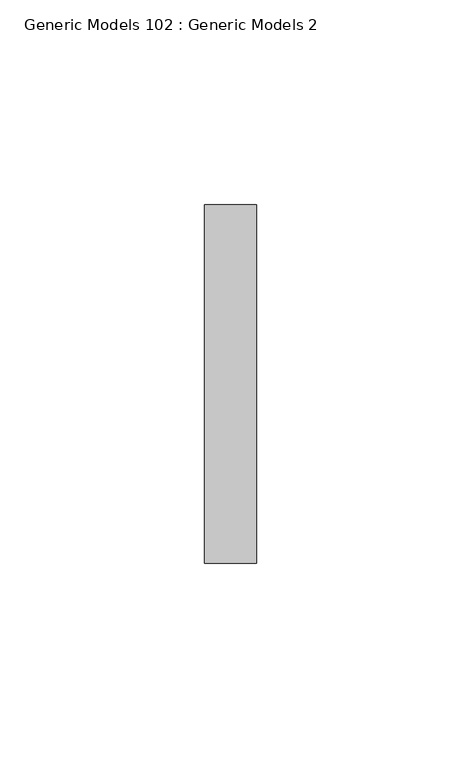
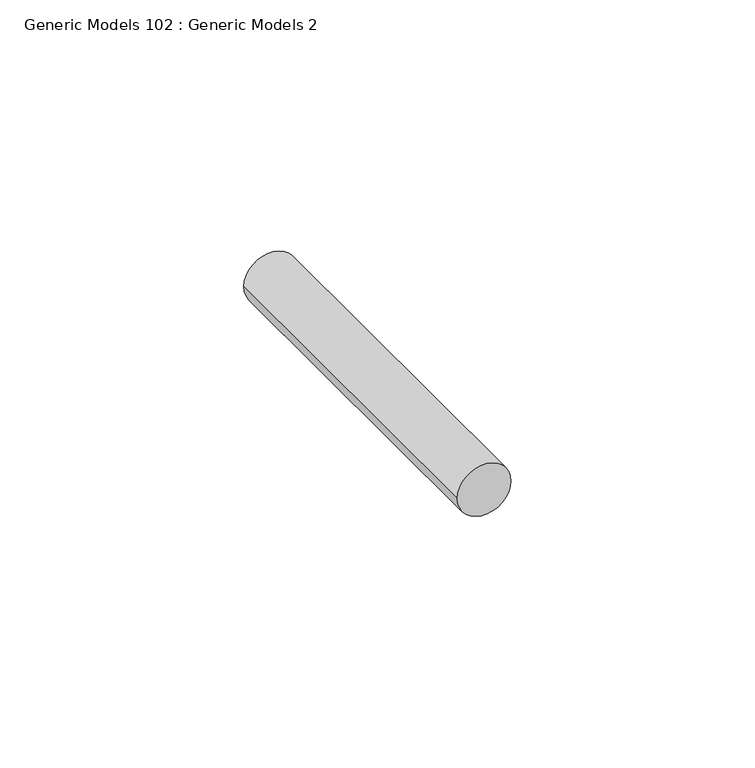
"""IFC4 building model written with IfcOpenShell, lengths in millimetres: proxy geometry, Generic Models 102 : Generic Models 2."""

from ifc_helpers import new_model, si_unit, point, frame, frame_2d, origin, place, context, project, spatial, circle_curve, trimmed, segment, composite_curve, outline, extrude, source, transform, mapped, element, save


def generic_models_102_generic_models_2_02627f47(model_context):
    return source(origin(), model_context, "Body", "SweptSolid", [
        extrude(outline(composite_curve([segment(trimmed(circle_curve(frame_2d((37345.8776334, 6010.5828124)), 6.35), [point((37345.8776334, 6004.2328124))], [point((37345.8776334, 6016.9328124))], False, "CARTESIAN"), True, "CONTINUOUS"), segment(trimmed(circle_curve(frame_2d((37345.8776334, 6010.5828124)), 6.35), [point((37345.8776334, 6016.9328124))], [point((37345.8776334, 6004.2328124))], False, "CARTESIAN"), True, "CONTINUOUS")], self_intersect=False)), frame((0.0, 1848.3666731, 0.0), z_axis=(0.0, 1.0, 0.0), x_axis=(0.0, 0.0, 1.0)), (0.0, 0.0, 1.0), 87.551022),
    ])


if __name__ == "__main__":
    model = new_model("IFC4")
    model_context = context("Model", 3, world=origin())
    ifc_project = project(units=[si_unit("LENGTHUNIT", "METRE", prefix="MILLI")], contexts=[model_context])
    site = spatial("IfcSite", under=ifc_project)
    building = spatial("IfcBuilding", under=site)
    placement = place(None, origin())
    generic_models_102_generic_models_2_shape = generic_models_102_generic_models_2_02627f47(model_context)
    element("IfcBuildingElementProxy", 1, Name="Generic Models 102 : Generic Models 2", ObjectType="Generic Models 102 : Generic Models 2", at=placement, inside=building, context=model_context, shape_type="MappedRepresentation", body=[
        mapped(generic_models_102_generic_models_2_shape, transform((0.0, 0.0, 0.0), x_axis=(1.0, 0.0, 0.0), y_axis=(0.0, 1.0, 0.0), z_axis=(0.0, 0.0, 1.0))),
    ])
    save(model, "model.ifc")

# Revit data of these elements
# Element 1 (IfcBuildingElementProxy, "Generic Models 102 : Generic Models 2")
#   Materials on its faces: "S.S. LAG BOLT - SEE STRUCT. DWGS"
# Materials
#   "S.S. LAG BOLT - SEE STRUCT. DWGS": class "Generic", colour RGB 120 120 120, transparency 0, Cost = 0
